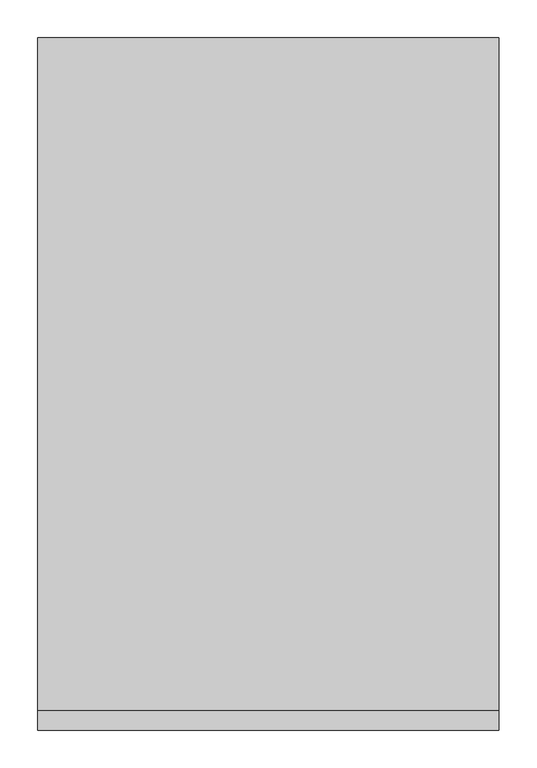
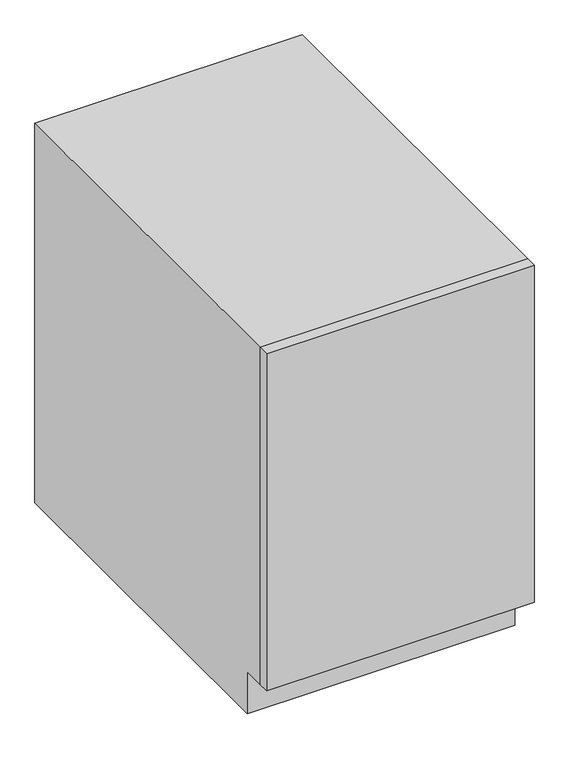
"""IFC4 building model written with IfcOpenShell, lengths in millimetres: furniture geometry, OD_CW_Base Cabinet : OD_CW_Base Cabinet."""

from ifc_helpers import new_model, si_unit, frame, origin, place, context, project, spatial, polyline, outline, extrude, source, transform, mapped, element, save


def furniture_b2d1dff0(model_context):
    return source(origin(), model_context, "Body", "SweptSolid", [
        extrude(outline(polyline([(18.7377049, -279.4), (628.3377049, -279.4), (628.3377049, -304.8), (18.7377049, -304.8), (18.7377049, -279.4)])), frame((0.0, 0.0, 101.6), z_axis=(0.0, 0.0, 1.0), x_axis=(1.0, 0.0, 0.0)), (0.0, 0.0, 1.0), 812.8),
        extrude(outline(polyline([(-279.4, 914.4), (609.6, 914.4), (609.6, 0.0), (-228.6, 0.0), (-228.6, 101.6), (-279.4, 101.6), (-279.4, 914.4)])), frame((18.7377049, 0.0, 0.0), z_axis=(1.0, 0.0, 0.0), x_axis=(0.0, 1.0, 0.0)), (0.0, 0.0, 1.0), 609.6),
    ])


if __name__ == "__main__":
    model = new_model("IFC4")
    model_context = context("Model", 3, world=origin())
    ifc_project = project(units=[si_unit("LENGTHUNIT", "METRE", prefix="MILLI")], contexts=[model_context])
    site = spatial("IfcSite", under=ifc_project)
    building = spatial("IfcBuilding", under=site)
    placement = place(None, origin())
    furniture_shape = furniture_b2d1dff0(model_context)
    element("IfcFurniture", 1, ObjectType="OD_CW_Base Cabinet : OD_CW_Base Cabinet", at=placement, inside=building, context=model_context, shape_type="MappedRepresentation", body=[
        mapped(furniture_shape, transform((0.0, 0.0, 0.0), x_axis=(1.0, 0.0, 0.0), y_axis=(0.0, 1.0, 0.0), z_axis=(0.0, 0.0, 1.0))),
    ])
    save(model, "model.ifc")

# Revit data of these elements
# Type "OD_CW_Base Cabinet : OD_CW_Base Cabinet"
#   OD_CW_Width [instance default] = 2' - 10"
#   OD_CW_Length [instance default] = 8' - 0"
#   OD_CW_Height [instance default] = 2' - 3"
#   Depth = 2' - 0"
#   Height = 3' - 0"
#   Width = 4' - 0"
#   OD_CW_Material_Front Panel [instance default] = none
#   OD_CW_Material_Body [instance default] = none
# Element 1 (IfcFurniture, "OD_CW_Base Cabinet : OD_CW_Base Cabinet")
#   OD_CW_Width = 3' - 0"
#   OD_CW_Length = 2' - 0"
#   OD_CW_Height = 3' - 0"
#   OD_CW_Material_Body = DESSERT FREEZER
#   Materials on its faces: "DESSERT FREEZER", "CASEWORK"
# Materials
#   "DESSERT FREEZER": class "Generic", colour RGB 187 187 187, transparency 0, Cost = 0
#   "CASEWORK": class "Generic", colour RGB 181 181 181, transparency 0, Cost = 0
